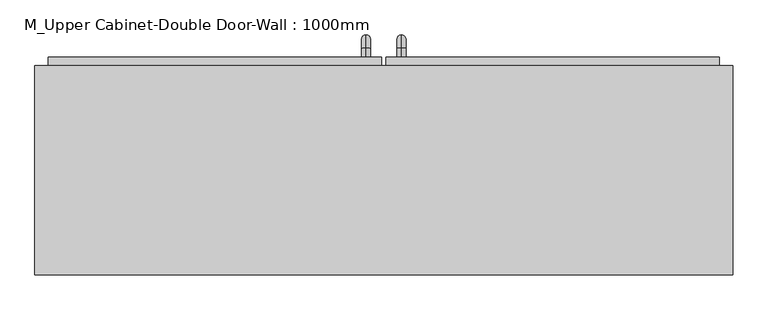
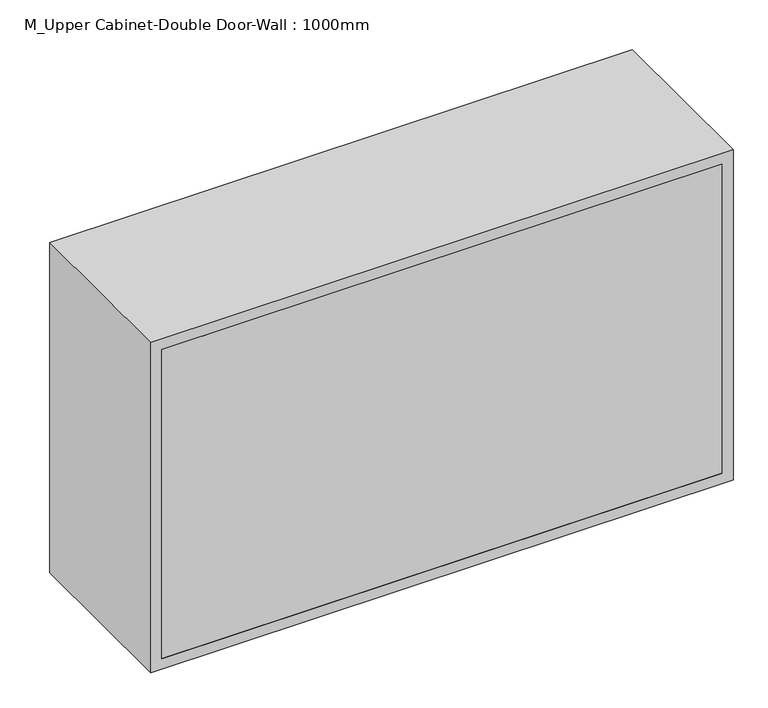
"""IFC4 building model written with IfcOpenShell, lengths in millimetres: furniture geometry, M_Upper Cabinet-Double Door-Wall : 1000mm."""

from ifc_helpers import new_model, si_unit, point, frame, origin, place, context, project, spatial, polyline, circle_curve, ellipse_curve, trimmed, outline, extrude, source, transform, mapped, element, save
from ifc_brep_helpers import plane_surface, cylinder_surface, revolved_surface, advanced_brep


def m_upper_cabinet_double_door_wall_1000mm_8ed99c58(model_context):
    return source(origin(), model_context, "Body", "SolidModel", [
        extrude(outline(polyline([(2000.0, -470.2288372), (1400.0, -470.2288372), (1400.0, 529.7711628), (2000.0, 529.7711628), (2000.0, -470.2288372)]), holes=[polyline([(1980.95, -451.1788372), (1980.95, 510.7211628), (1419.05, 510.7211628), (1419.05, -451.1788372), (1980.95, -451.1788372)])]), frame((0.0, 75.0, 0.0), z_axis=(0.0, 1.0, 0.0), x_axis=(0.0, 0.0, 1.0)), (0.0, 0.0, 1.0), 300.0),
        extrude(outline(polyline([(510.7211628, 75.0), (-451.1788372, 75.0), (-451.1788372, 94.05), (510.7211628, 94.05), (510.7211628, 75.0)])), frame((0.0, 0.0, 1419.05), z_axis=(0.0, 0.0, 1.0), x_axis=(1.0, 0.0, 0.0)), (0.0, 0.0, 1.0), 561.9),
        extrude(outline(polyline([(32.9461628, 387.7), (510.7211628, 387.7), (510.7211628, 355.95), (32.9461628, 355.95), (32.9461628, 387.7)])), frame((0.0, 0.0, 1419.05), z_axis=(0.0, 0.0, 1.0), x_axis=(1.0, 0.0, 0.0)), (0.0, 0.0, 1.0), 561.9),
        extrude(outline(polyline([(-451.1788372, 387.7), (26.5961628, 387.7), (26.5961628, 355.95), (-451.1788372, 355.95), (-451.1788372, 387.7)])), frame((0.0, 0.0, 1419.05), z_axis=(0.0, 0.0, 1.0), x_axis=(1.0, 0.0, 0.0)), (0.0, 0.0, 1.0), 561.9),
        advanced_brep(
        [(4.3711628, 387.7, 1546.05), (4.3711628, 387.7, 1558.75), (4.3711628, 400.4, 1546.05), (4.3711628, 400.4, 1558.75), (4.3711628, 419.45, 1539.7), (4.3711628, 406.75, 1539.7), (4.3711628, 406.75, 1463.5), (4.3711628, 419.45, 1463.5), (4.3711628, 400.4, 1444.45), (4.3711628, 400.4, 1457.15), (4.3711628, 387.7, 1457.15), (4.3711628, 387.7, 1444.45)],
        [
            (0, 1, circle_curve(frame((4.3711628, 387.7, 1552.4), z_axis=(0.0, -1.0, 0.0), x_axis=(0.0, 0.0, 1.0)), 6.35)),
            (1, 0, circle_curve(frame((4.3711628, 387.7, 1552.4), z_axis=(0.0, -1.0, 0.0), x_axis=(0.0, 0.0, 1.0)), 6.35)),
            (0, 2),
            (2, 3, circle_curve(frame((4.3711628, 400.4, 1552.4), z_axis=(0.0, -1.0, 0.0), x_axis=(0.0, 0.0, 1.0)), 6.35)),
            (3, 1),
            (3, 2, circle_curve(frame((4.3711628, 400.4, 1552.4), z_axis=(0.0, -1.0, 0.0), x_axis=(0.0, 0.0, 1.0)), 6.35)),
            (4, 3, circle_curve(frame((4.3711628, 400.4, 1539.7), z_axis=(1.0, 0.0, 0.0), x_axis=(0.0, 0.0, 1.0)), 19.05)),
            (2, 5, circle_curve(frame((4.3711628, 400.4, 1539.7), z_axis=(-1.0, 0.0, 0.0), x_axis=(0.0, 0.0, 1.0)), 6.35)),
            (5, 4, circle_curve(frame((4.3711628, 413.1, 1539.7), z_axis=(0.0, 0.0, 1.0), x_axis=(0.0, 1.0, 0.0)), 6.35)),
            (4, 5, circle_curve(frame((4.3711628, 413.1, 1539.7), z_axis=(0.0, 0.0, 1.0), x_axis=(0.0, 1.0, 0.0)), 6.35)),
            (5, 6),
            (6, 7, circle_curve(frame((4.3711628, 413.1, 1463.5), z_axis=(0.0, 0.0, 1.0), x_axis=(0.0, 1.0, 0.0)), 6.35)),
            (7, 4),
            (7, 6, circle_curve(frame((4.3711628, 413.1, 1463.5), z_axis=(0.0, 0.0, 1.0), x_axis=(0.0, 1.0, 0.0)), 6.35)),
            (8, 7, circle_curve(frame((4.3711628, 400.4, 1463.5), z_axis=(1.0, 0.0, 0.0), x_axis=(0.0, 1.0, 0.0)), 19.05)),
            (6, 9, circle_curve(frame((4.3711628, 400.4, 1463.5), z_axis=(-1.0, 0.0, 0.0), x_axis=(0.0, 1.0, 0.0)), 6.35)),
            (9, 8, circle_curve(frame((4.3711628, 400.4, 1450.8), z_axis=(0.0, 1.0, 0.0), x_axis=(0.0, 0.0, -1.0)), 6.35)),
            (8, 9, circle_curve(frame((4.3711628, 400.4, 1450.8), z_axis=(0.0, 1.0, 0.0), x_axis=(0.0, 0.0, -1.0)), 6.35)),
            (10, 11, circle_curve(frame((4.3711628, 387.7, 1450.8), z_axis=(0.0, -1.0, 0.0), x_axis=(0.0, 0.0, -1.0)), 6.35)),
            (11, 10, circle_curve(frame((4.3711628, 387.7, 1450.8), z_axis=(0.0, -1.0, 0.0), x_axis=(0.0, 0.0, -1.0)), 6.35)),
            (9, 10),
            (11, 8),
        ],
        [
            plane_surface(frame((-1.9788372, 387.7, 1552.4), z_axis=(0.0, -1.0, 0.0), x_axis=(0.0, 0.0, 1.0))),
            cylinder_surface(frame((4.3711628, 387.7, 1552.4), z_axis=(0.0, -1.0, 0.0), x_axis=(0.0, 0.0, 1.0)), 6.35),
            revolved_surface(trimmed(ellipse_curve(frame((4.3711628, 400.4, 1552.4), z_axis=(0.0, -1.0, 0.0), x_axis=(0.0, 0.0, 1.0)), 6.35, 6.35), [point((4.3711628, 400.4, 1546.05))], [point((4.3711628, 400.4, 1558.75))], True, "CARTESIAN"), (4.3711628, 400.4, 1539.7), (-1.0, 0.0, 0.0)),
            revolved_surface(trimmed(ellipse_curve(frame((4.3711628, 400.4, 1552.4), z_axis=(0.0, -1.0, 0.0), x_axis=(0.0, 0.0, 1.0)), 6.35, 6.35), [point((4.3711628, 400.4, 1558.75))], [point((4.3711628, 400.4, 1546.05))], True, "CARTESIAN"), (4.3711628, 400.4, 1539.7), (-1.0, 0.0, 0.0)),
            cylinder_surface(frame((4.3711628, 413.1, 1539.7), z_axis=(0.0, 0.0, 1.0), x_axis=(0.0, 1.0, 0.0)), 6.35),
            revolved_surface(trimmed(ellipse_curve(frame((4.3711628, 413.1, 1463.5), z_axis=(0.0, 0.0, 1.0), x_axis=(0.0, 1.0, 0.0)), 6.35, 6.35), [point((4.3711628, 406.75, 1463.5))], [point((4.3711628, 419.45, 1463.5))], True, "CARTESIAN"), (4.3711628, 400.4, 1463.5), (-1.0, 0.0, 0.0)),
            revolved_surface(trimmed(ellipse_curve(frame((4.3711628, 413.1, 1463.5), z_axis=(0.0, 0.0, 1.0), x_axis=(0.0, 1.0, 0.0)), 6.35, 6.35), [point((4.3711628, 419.45, 1463.5))], [point((4.3711628, 406.75, 1463.5))], True, "CARTESIAN"), (4.3711628, 400.4, 1463.5), (-1.0, 0.0, 0.0)),
            plane_surface(frame((-1.9788372, 387.7, 1450.8), z_axis=(0.0, -1.0, 0.0), x_axis=(0.0, 0.0, -1.0))),
            cylinder_surface(frame((4.3711628, 400.4, 1450.8), z_axis=(0.0, 1.0, 0.0), x_axis=(0.0, 0.0, -1.0)), 6.35),
        ],
        [
            (0, [[1, 2]]),
            (1, [[-1, 3, 4, 5]]),
            (1, [[-2, -5, 6, -3]]),
            (2, [[7, -4, 8, 9]]),
            (3, [[-8, -6, -7, 10]]),
            (4, [[-9, 11, 12, 13]]),
            (4, [[-10, -13, 14, -11]]),
            (5, [[15, -12, 16, 17]]),
            (6, [[-16, -14, -15, 18]]),
            (7, [[19, 20]]),
            (8, [[-17, 21, -20, 22]]),
            (8, [[-18, -22, -19, -21]]),
        ],
    ),
        advanced_brep(
        [(55.1711628, 387.7, 1546.05), (55.1711628, 387.7, 1558.75), (55.1711628, 400.4, 1546.05), (55.1711628, 400.4, 1558.75), (55.1711628, 419.45, 1539.7), (55.1711628, 406.75, 1539.7), (55.1711628, 406.75, 1463.5), (55.1711628, 419.45, 1463.5), (55.1711628, 400.4, 1444.45), (55.1711628, 400.4, 1457.15), (55.1711628, 387.7, 1457.15), (55.1711628, 387.7, 1444.45)],
        [
            (0, 1, circle_curve(frame((55.1711628, 387.7, 1552.4), z_axis=(0.0, -1.0, 0.0), x_axis=(0.0, 0.0, -1.0)), 6.35)),
            (1, 0, circle_curve(frame((55.1711628, 387.7, 1552.4), z_axis=(0.0, -1.0, 0.0), x_axis=(0.0, 0.0, -1.0)), 6.35)),
            (0, 2),
            (2, 3, circle_curve(frame((55.1711628, 400.4, 1552.4), z_axis=(0.0, -1.0, 0.0), x_axis=(0.0, 0.0, -1.0)), 6.35)),
            (3, 1),
            (3, 2, circle_curve(frame((55.1711628, 400.4, 1552.4), z_axis=(0.0, -1.0, 0.0), x_axis=(0.0, 0.0, -1.0)), 6.35)),
            (4, 3, circle_curve(frame((55.1711628, 400.4, 1539.7), z_axis=(1.0, 0.0, 0.0), x_axis=(0.0, 0.0, 1.0)), 19.05)),
            (2, 5, circle_curve(frame((55.1711628, 400.4, 1539.7), z_axis=(-1.0, 0.0, 0.0), x_axis=(0.0, 0.0, 1.0)), 6.35)),
            (5, 4, circle_curve(frame((55.1711628, 413.1, 1539.7), z_axis=(0.0, 0.0, 1.0), x_axis=(0.0, -1.0, 0.0)), 6.35)),
            (4, 5, circle_curve(frame((55.1711628, 413.1, 1539.7), z_axis=(0.0, 0.0, 1.0), x_axis=(0.0, -1.0, 0.0)), 6.35)),
            (5, 6),
            (6, 7, circle_curve(frame((55.1711628, 413.1, 1463.5), z_axis=(0.0, 0.0, 1.0), x_axis=(0.0, -1.0, 0.0)), 6.35)),
            (7, 4),
            (7, 6, circle_curve(frame((55.1711628, 413.1, 1463.5), z_axis=(0.0, 0.0, 1.0), x_axis=(0.0, -1.0, 0.0)), 6.35)),
            (8, 7, circle_curve(frame((55.1711628, 400.4, 1463.5), z_axis=(1.0, 0.0, 0.0), x_axis=(0.0, 1.0, 0.0)), 19.05)),
            (6, 9, circle_curve(frame((55.1711628, 400.4, 1463.5), z_axis=(-1.0, 0.0, 0.0), x_axis=(0.0, 1.0, 0.0)), 6.35)),
            (9, 8, circle_curve(frame((55.1711628, 400.4, 1450.8), z_axis=(0.0, 1.0, 0.0), x_axis=(0.0, 0.0, 1.0)), 6.35)),
            (8, 9, circle_curve(frame((55.1711628, 400.4, 1450.8), z_axis=(0.0, 1.0, 0.0), x_axis=(0.0, 0.0, 1.0)), 6.35)),
            (10, 11, circle_curve(frame((55.1711628, 387.7, 1450.8), z_axis=(0.0, -1.0, 0.0), x_axis=(0.0, 0.0, 1.0)), 6.35)),
            (11, 10, circle_curve(frame((55.1711628, 387.7, 1450.8), z_axis=(0.0, -1.0, 0.0), x_axis=(0.0, 0.0, 1.0)), 6.35)),
            (9, 10),
            (11, 8),
        ],
        [
            plane_surface(frame((48.8211628, 387.7, 1552.4), z_axis=(0.0, -1.0, 0.0), x_axis=(0.0, 0.0, 1.0))),
            cylinder_surface(frame((55.1711628, 387.7, 1552.4), z_axis=(0.0, -1.0, 0.0), x_axis=(0.0, 0.0, -1.0)), 6.35),
            revolved_surface(trimmed(ellipse_curve(frame((55.1711628, 400.4, 1552.4), z_axis=(0.0, -1.0, 0.0), x_axis=(0.0, 0.0, -1.0)), 6.35, 6.35), [point((55.1711628, 400.4, 1546.05))], [point((55.1711628, 400.4, 1558.75))], True, "CARTESIAN"), (55.1711628, 400.4, 1539.7), (-1.0, 0.0, 0.0)),
            revolved_surface(trimmed(ellipse_curve(frame((55.1711628, 400.4, 1552.4), z_axis=(0.0, -1.0, 0.0), x_axis=(0.0, 0.0, -1.0)), 6.35, 6.35), [point((55.1711628, 400.4, 1558.75))], [point((55.1711628, 400.4, 1546.05))], True, "CARTESIAN"), (55.1711628, 400.4, 1539.7), (-1.0, 0.0, 0.0)),
            cylinder_surface(frame((55.1711628, 413.1, 1539.7), z_axis=(0.0, 0.0, 1.0), x_axis=(0.0, -1.0, 0.0)), 6.35),
            revolved_surface(trimmed(ellipse_curve(frame((55.1711628, 413.1, 1463.5), z_axis=(0.0, 0.0, 1.0), x_axis=(0.0, -1.0, 0.0)), 6.35, 6.35), [point((55.1711628, 406.75, 1463.5))], [point((55.1711628, 419.45, 1463.5))], True, "CARTESIAN"), (55.1711628, 400.4, 1463.5), (-1.0, 0.0, 0.0)),
            revolved_surface(trimmed(ellipse_curve(frame((55.1711628, 413.1, 1463.5), z_axis=(0.0, 0.0, 1.0), x_axis=(0.0, -1.0, 0.0)), 6.35, 6.35), [point((55.1711628, 419.45, 1463.5))], [point((55.1711628, 406.75, 1463.5))], True, "CARTESIAN"), (55.1711628, 400.4, 1463.5), (-1.0, 0.0, 0.0)),
            plane_surface(frame((48.8211628, 387.7, 1450.8), z_axis=(0.0, -1.0, 0.0), x_axis=(0.0, 0.0, -1.0))),
            cylinder_surface(frame((55.1711628, 400.4, 1450.8), z_axis=(0.0, 1.0, 0.0), x_axis=(0.0, 0.0, 1.0)), 6.35),
        ],
        [
            (0, [[1, 2]]),
            (1, [[-1, 3, 4, 5]]),
            (1, [[-2, -5, 6, -3]]),
            (2, [[7, -4, 8, 9]]),
            (3, [[-8, -6, -7, 10]]),
            (4, [[-9, 11, 12, 13]]),
            (4, [[-10, -13, 14, -11]]),
            (5, [[15, -12, 16, 17]]),
            (6, [[-16, -14, -15, 18]]),
            (7, [[19, 20]]),
            (8, [[-17, 21, -20, 22]]),
            (8, [[-18, -22, -19, -21]]),
        ],
    ),
    ])


if __name__ == "__main__":
    model = new_model("IFC4")
    model_context = context("Model", 3, world=origin())
    ifc_project = project(units=[si_unit("LENGTHUNIT", "METRE", prefix="MILLI")], contexts=[model_context])
    site = spatial("IfcSite", under=ifc_project)
    building = spatial("IfcBuilding", under=site)
    placement = place(None, origin())
    m_upper_cabinet_double_door_wall_1000mm_shape = m_upper_cabinet_double_door_wall_1000mm_8ed99c58(model_context)
    element("IfcFurniture", 1, ObjectType="M_Upper Cabinet-Double Door-Wall : 1000mm", at=placement, inside=building, context=model_context, shape_type="MappedRepresentation", body=[
        mapped(m_upper_cabinet_double_door_wall_1000mm_shape, transform((0.0, 0.0, 0.0), x_axis=(1.0, 0.0, 0.0), y_axis=(0.0, 1.0, 0.0), z_axis=(0.0, 0.0, 1.0))),
    ])
    save(model, "model.ifc")

# Revit data of these elements
# Project information
#   Organization Name = "Organization Name"
#   Organization Description = "Organization Description"
#   Building Name = "Building Name"
#   Project Issue Date = "Issue Date"
#   Project Status = "Project Status"
#   Client Name = "Client Name"
#   Project Address = "Enter address here\nAddress Line 2"
#   Project Name = "Project Name"
#   Project Number = "Project Number"
# Type "M_Upper Cabinet-Double Door-Wall : 1000mm"
#   Depth = 300 mm
#   Height = 600 mm
#   Top Of Cabinet = 2000 mm
#   Width = 1000 mm
#   Cabinet Material = none
#   Door/Drawer Material = none
#   Handle Material = Cabinets - Handles
#   Default Elevation = 0
# Element 1 (IfcFurniture, "M_Upper Cabinet-Double Door-Wall : 1000mm")
#   Materials on its faces: "Cabinets", "Cabinets - Handles"
# Materials
#   "Cabinets - Handles": class "Metal", colour RGB 57 57 57, transparency 0, Cost = 0
#   "Cabinets": class "Miscellaneous", colour RGB 249 249 249, transparency 0, Cost = 0
